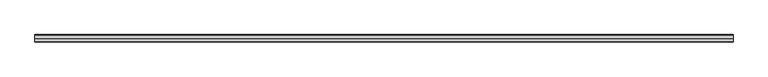
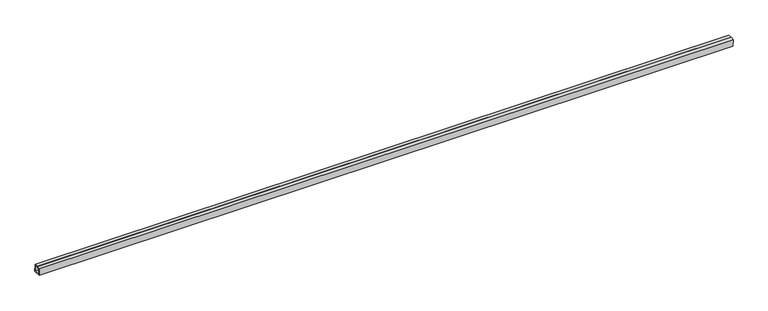
"""IFC4 building model written with IfcOpenShell, lengths in millimetres: proxy geometry, Inner panel:Inner panel:1:Inner panel:1 : Inner panel:Inner panel:300324:2:Inner panel:1:Inner panel:1 : Inner panel:Inner panel:300324:2 : Inner panel:Inner panel:1:Inner panel:1 : Inner panel:Inner panel:300324:300043:39 : Inner panel:Inner panel:1:Inner panel:1 : Inner panel:Inner panel:300324:2:Inner panel:1:Inner panel:1 : Inner panel:Inner panel:300324:2 : Inner panel:Inner panel:1:Inner panel:1 : Inner panel:Inner panel:300324:300043:308120."""

from ifc_helpers import new_model, si_unit, frame, origin, place, context, project, spatial, polyline, outline, extrude, source, transform, mapped, element, save


def generic_models_3d34534d(model_context):
    return source(origin(), model_context, "Body", "SweptSolid", [
        extrude(outline(polyline([(-580481.3921913, 3888.2024845), (-580463.1517681, 3888.9625021), (-580461.5656444, 3850.895532), (-580499.6326145, 3849.3094083), (-580501.2187382, 3887.3763783), (-580482.9783151, 3888.136396), (-580482.8791823, 3885.7572103), (-580498.7404199, 3885.0963254), (-580497.3525616, 3851.7877266), (-580464.0439628, 3853.1755849), (-580465.431821, 3886.4841837), (-580481.2930586, 3885.8232988), (-580481.3921913, 3888.2024845)])), frame((612749.9867239, 0.0, 0.0), z_axis=(1.0, 0.0, 0.0), x_axis=(0.0, 1.0, 0.0)), (0.0, 0.0, 1.0), 3657.6),
    ])


if __name__ == "__main__":
    model = new_model("IFC4")
    model_context = context("Model", 3, world=origin())
    ifc_project = project(units=[si_unit("LENGTHUNIT", "METRE", prefix="MILLI")], contexts=[model_context])
    site = spatial("IfcSite", under=ifc_project)
    building = spatial("IfcBuilding", under=site)
    placement = place(None, origin())
    generic_models_shape = generic_models_3d34534d(model_context)
    element("IfcBuildingElementProxy", 1, Name="Inner panel:Inner panel:1:Inner panel:1 : Inner panel:Inner panel:300324:2:Inner panel:1:Inner panel:1 : Inner panel:Inner panel:300324:2 : Inner panel:Inner panel:1:Inner panel:1 : Inner panel:Inner panel:300324:300043:39 : Inner panel:Inner panel:1:Inner panel:1 : Inner panel:Inner panel:300324:2:Inner panel:1:Inner panel:1 : Inner panel:Inner panel:300324:2 : Inner panel:Inner panel:1:Inner panel:1 : Inner panel:Inner panel:300324:300043:308120", ObjectType="Inner panel:Inner panel:1:Inner panel:1 : Inner panel:Inner panel:300324:2:Inner panel:1:Inner panel:1 : Inner panel:Inner panel:300324:2 : Inner panel:Inner panel:1:Inner panel:1 : Inner panel:Inner panel:300324:300043:39 : Inner panel:Inner panel:1:Inner panel:1 : Inner panel:Inner panel:300324:2:Inner panel:1:Inner panel:1 : Inner panel:Inner panel:300324:2 : Inner panel:Inner panel:1:Inner panel:1 : Inner panel:Inner panel:300324:300043:308120", at=placement, inside=building, context=model_context, shape_type="MappedRepresentation", body=[
        mapped(generic_models_shape, transform((0.0, 0.0, 0.0), x_axis=(1.0, 0.0, 0.0), y_axis=(0.0, 1.0, 0.0), z_axis=(0.0, 0.0, 1.0))),
    ])
    save(model, "model.ifc")

# Revit data of these elements
# Type "Inner panel:Inner panel:1:Inner panel:1 : Inner panel:Inner panel:300324:2:Inner panel:1:Inner panel:1 : Inner panel:Inner panel:300324:2 : Inner panel:Inner panel:1:Inner panel:1 : Inner panel:Inner panel:300324:300043:39 : Inner panel:Inner panel:1:Inner panel:1 : Inner panel:Inner panel:300324:2:Inner panel:1:Inner panel:1 : Inner panel:Inner panel:300324:2 : Inner panel:Inner panel:1:Inner panel:1 : Inner panel:Inner panel:300324:300043:308120"
#   NameOverride = "Inner panel:Inner panel:1:Inner panel:1 : Inner panel:Inner panel:300324:2:Inner panel:1:Inner panel:1 : Inner panel:Inner panel:300324:2 : Inner panel:Inner panel:1:Inner panel:1 : Inner panel:Inner panel:300324:300043:308120"
#   ObjectTypeOverride = "Inner panel:1:Inner panel:1 : Inner panel:Inner panel:300324:2 : Inner panel:Inner panel:1:Inner panel:1 : Inner panel:Inner panel:300324:300043"
#   Reference = "Inner panel"
#   Tag = "308120"
# Element 1 (IfcBuildingElementProxy, "Inner panel:Inner panel:1:Inner panel:1 : Inner panel:Inner panel:300324:2:Inner panel:1:Inner panel:1 : Inner panel:Inner panel:300324:2 : Inner panel:Inner panel:1:Inner panel:1 : Inner panel:Inner panel:300324:300043:39 : Inner panel:Inner panel:1:Inner panel:1 : Inner panel:Inner panel:300324:2:Inner panel:1:Inner panel:1 : Inner panel:Inner panel:300324:2 : Inner panel:Inner panel:1:Inner panel:1 : Inner panel:Inner panel:300324:300043:308120")
#   Materials on its faces: "1 1/2\" X 1 1/2\" SPLIT-SEAM SQUARE TUBING (~24\" CANTILEVER FROM C.L. OF GLULAM)"
# Materials
#   "1 1/2\" X 1 1/2\" SPLIT-SEAM SQUARE TUBING (~24\" CANTILEVER FROM C.L. OF GLULAM)": class "Unassigned", colour RGB 202 201 200, transparency 0, Cost = 0
